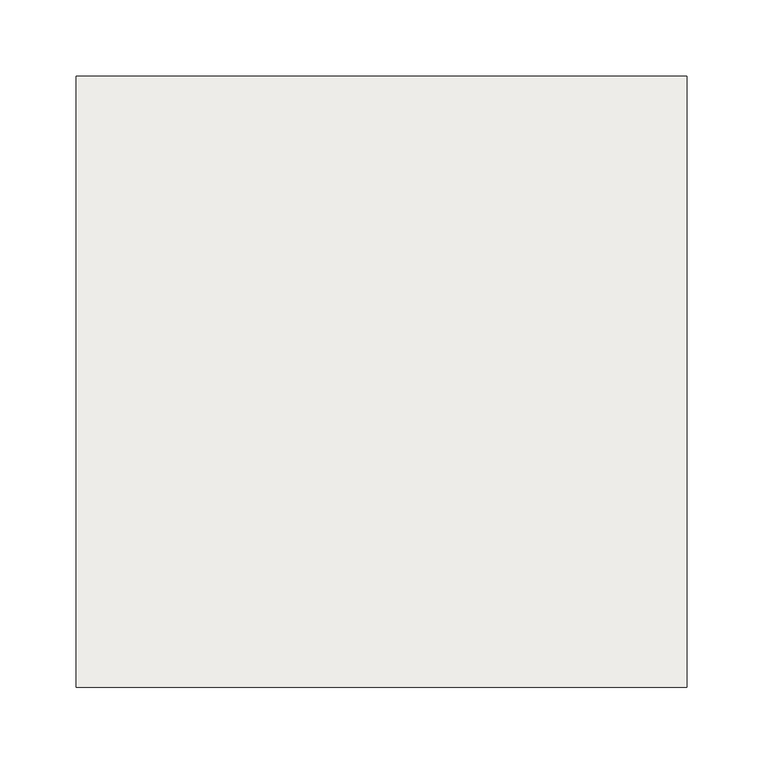
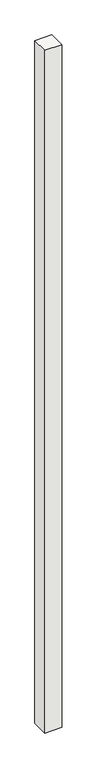
"""IFC4 building model written with IfcOpenShell, lengths in millimetres: slab geometry, NLRS_17_SFO_TLB_funderingspaal geheid beton prefab-AV-MMBPC_gen_rsf : heipaal beton prefab_gen__bxh 400x400."""

from ifc_helpers import new_model, si_unit, frame, origin, place, context, project, spatial, polyline, outline, extrude, source, transform, mapped, element, save


def slab_f9187350(model_context):
    return source(origin(), model_context, "Body", "SweptSolid", [
        extrude(outline(polyline([(200.0, -200.0), (-200.0, -200.0), (-200.0, 200.0), (200.0, 200.0), (200.0, -200.0)])), frame((0.0, 0.0, -20000.0), z_axis=(0.0, 0.0, 1.0), x_axis=(1.0, 0.0, 0.0)), (0.0, 0.0, 1.0), 16925.0),
    ])


if __name__ == "__main__":
    model = new_model("IFC4")
    model_context = context("Model", 3, world=origin())
    ifc_project = project(units=[si_unit("LENGTHUNIT", "METRE", prefix="MILLI")], contexts=[model_context])
    site = spatial("IfcSite", under=ifc_project)
    building = spatial("IfcBuilding", under=site)
    placement = place(None, origin())
    slab_shape = slab_f9187350(model_context)
    element("IfcSlab", 1, ObjectType="NLRS_17_SFO_TLB_funderingspaal geheid beton prefab-AV-MMBPC_gen_rsf : heipaal beton prefab_gen__bxh 400x400", at=placement, inside=building, context=model_context, shape_type="MappedRepresentation", body=[
        mapped(slab_shape, transform((0.0, 0.0, 0.0), x_axis=(1.0, 0.0, 0.0), y_axis=(0.0, 1.0, 0.0), z_axis=(0.0, 0.0, 1.0))),
    ])
    save(model, "model.ifc")

# Revit data of these elements
# Type "NLRS_17_SFO_TLB_funderingspaal geheid beton prefab-AV-MMBPC_gen_rsf : heipaal beton prefab_gen__bxh 400x400"
#   Export Type to IFC As = "IfcPile"
#   Type IfcGUID = "10$Kfo5uPCAOPJEOo5LE_W"
#   Type Comments = "prefab heipaal 400x400"
#   Model = " "
#   Manufacturer = " "
#   Description = "prefab heipaal 400x400"
#   Assembly Code = "17.21"
#   Width = 400 mm
#   Slanted Angle [instance default] = 0.00°
#   NLRS_S_draagvermogen_trek [instance default] = 0.00 kN
#   NLRS_S_draagvermogen_druk [instance default] = 0.00 kN
#   NLRS_C_lengte [instance default] = 1660 mm
#   NLRS_C_hoogte = 400 mm
#   NLRS_C_breedte = 400 mm
#   Height [instance default] = 1660 mm
#   Length [instance default] = 1660 mm
#   Angle [instance default] = 0.00°
#   Slanted [instance default] = 0
#   Structural Material = NLRS_f2_beton prefab_gen_rsf
#   Keynote = ""
# Element 1 (IfcSlab, "NLRS_17_SFO_TLB_funderingspaal geheid beton prefab-AV-MMBPC_gen_rsf : heipaal beton prefab_gen__bxh 400x400")
#   NLRS_C_lengte = 16925 mm
#   Height = 16925 mm
#   Length = 16925 mm
#   Materials on its faces: "NLRS_f2_beton prefab_gen_rsf"
# Materials
#   "NLRS_f2_beton prefab_gen_rsf": class "F - Niet gebakken kunststeen", colour RGB 129 133 118, transparency 0, Keynote = "f2", Manufacturer = "Revit Standards Foundation", URL = "www.revitstandards.org", Description = "beton prefab", Cost = 0
